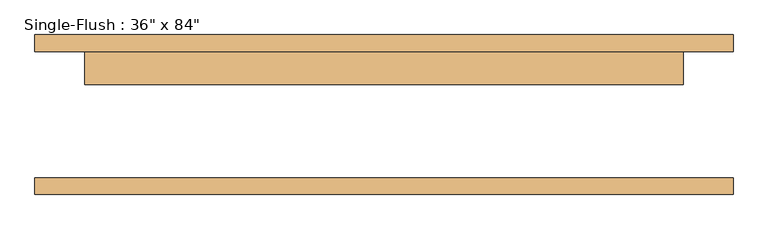
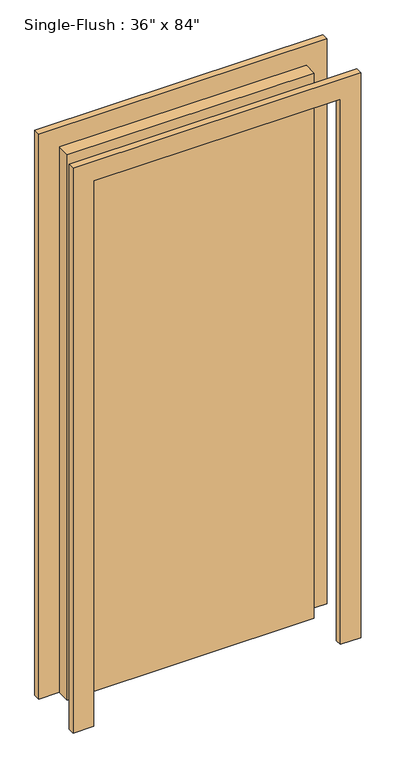
"""IFC4 building model written with IfcOpenShell, lengths in millimetres: door geometry."""

from ifc_helpers import new_model, si_unit, frame, origin, origin_with_axes, place, context, project, spatial, polyline, outline, extrude, source, transform, mapped, element, save


def door_d6d25fb4(model_context):
    return source(origin(), model_context, "Body", "SweptSolid", [
        extrude(outline(polyline([(2209.8, -533.4), (0.0, -533.4), (0.0, -457.2), (2133.6, -457.2), (2133.6, 457.2), (0.0, 457.2), (0.0, 533.4), (2209.8, 533.4), (2209.8, -533.4)])), frame((0.0, 96.8375, 0.0), z_axis=(0.0, 1.0, 0.0), x_axis=(0.0, 0.0, 1.0)), (0.0, 0.0, 1.0), 25.4),
        extrude(outline(polyline([(2209.8, 533.4), (2209.8, -533.4), (0.0, -533.4), (0.0, -457.2), (2133.6, -457.2), (2133.6, 457.2), (0.0, 457.2), (0.0, 533.4), (2209.8, 533.4)])), frame((0.0, -122.2375, 0.0), z_axis=(0.0, 1.0, 0.0), x_axis=(0.0, 0.0, 1.0)), (0.0, 0.0, 1.0), 25.4),
        extrude(outline(polyline([(457.2, 46.0375), (-457.2, 46.0375), (-457.2, 96.8375), (457.2, 96.8375), (457.2, 46.0375)])), origin_with_axes(), (0.0, 0.0, 1.0), 2133.6),
    ])


if __name__ == "__main__":
    model = new_model("IFC4")
    model_context = context("Model", 3, world=origin())
    ifc_project = project(units=[si_unit("LENGTHUNIT", "METRE", prefix="MILLI")], contexts=[model_context])
    site = spatial("IfcSite", under=ifc_project)
    building = spatial("IfcBuilding", under=site)
    placement = place(None, origin())
    door_shape = door_d6d25fb4(model_context)
    element("IfcDoor", 1, ObjectType="Single-Flush : 36\" x 84\"", at=placement, inside=building, context=model_context, shape_type="MappedRepresentation", body=[
        mapped(door_shape, transform((0.0, 0.0, 0.0), x_axis=(1.0, 0.0, 0.0), y_axis=(0.0, 1.0, 0.0), z_axis=(0.0, 0.0, 1.0))),
    ])
    save(model, "model.ifc")

# Revit data of these elements
# Type "Single-Flush : 36\" x 84\""
#   Type Mark = "1"
#   Assembly Code = "C1020"
#   Thickness = 0' - 2"
#   Height = 7' - 0"
#   Trim Projection Ext = 0' - 1"
#   Trim Projection Int = 0' - 1"
#   Trim Width = 0' - 3"
#   Width = 3' - 0"
#   Door Material = none
#   Frame Material = none
#   Function = (empty or 0)
#   Wall Closure = (empty or 0)
